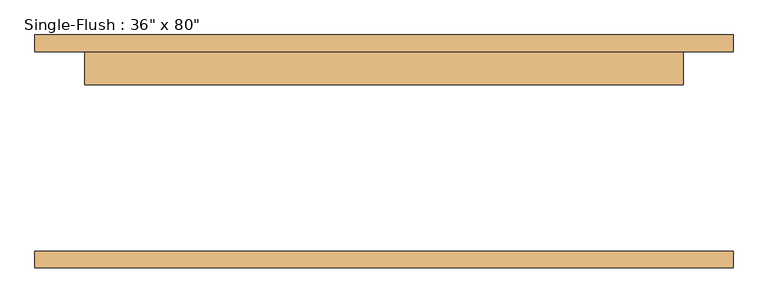
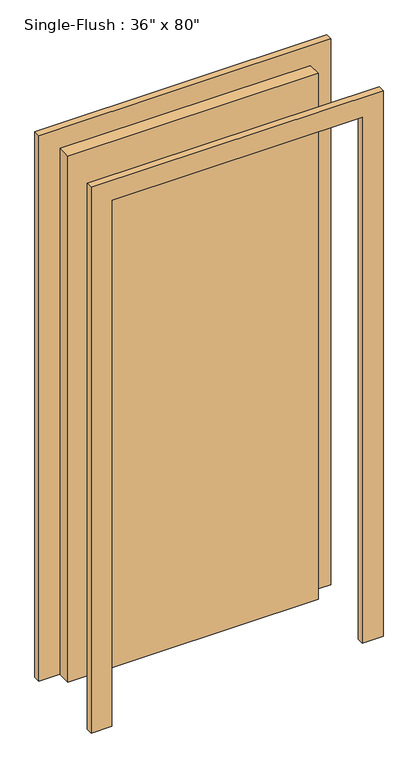
"""IFC4 building model written with IfcOpenShell, lengths in millimetres: door geometry."""

import ifcopenshell
import ifcopenshell.guid

model = None  # the IFC model being written
_history = None  # IfcOwnerHistory: only IFC2X3 demands one
_inside = {}  # id of a spatial element -> (the spatial element, [elements in it])
_under = {}  # id of a project, library or spatial element -> (it, [spatial elements below it])
_declared = {}  # id of a project -> (the project, [libraries it declares])
_typed = {}  # id of a type object -> (the type object, [elements of that type])
_made_of = {}  # id of a material, layer set ... -> (it, [elements and type objects made of it])


def new_model(schema):
    """Start an empty IFC model of exactly this schema.

    Asked for "IFC4X3", IfcOpenShell would pick the latest addendum, in which some entities
    have other attributes; the version numbers below select the first issue.
    IFC2X3 requires an IfcOwnerHistory on every rooted entity: one is made here for all.
    """
    global model, _history
    if schema == "IFC4X3":
        model = ifcopenshell.file(schema_version=(4, 3, 0, 0))
    else:
        model = ifcopenshell.file(schema=schema)
    _inside.clear()
    _under.clear()
    _declared.clear()
    _typed.clear()
    _made_of.clear()
    _history = None
    if model.schema == "IFC2X3":
        org = make("IfcOrganization", Name="unknown")
        user = make(
            "IfcPersonAndOrganization",
            ThePerson=make("IfcPerson", FamilyName="unknown"),
            TheOrganization=org,
        )
        app = make(
            "IfcApplication",
            ApplicationDeveloper=org,
            Version="unknown",
            ApplicationFullName="unknown",
            ApplicationIdentifier="unknown",
        )
        _history = make(
            "IfcOwnerHistory",
            OwningUser=user,
            OwningApplication=app,
            ChangeAction="ADDED",
            CreationDate=0,
        )
    return model


def make(cls, **values):
    """One entity of the class cls with the attributes given. An attribute that is None is left unset."""
    return model.create_entity(
        cls, **{name: value for name, value in values.items() if value is not None}
    )


def rooted(cls, **values):
    """An entity with a GlobalId (a new one), such as an element, a storey or a relation."""
    return make(cls, GlobalId=ifcopenshell.guid.new(), OwnerHistory=_history, **values)


def si_unit(unit_type, name, prefix=None):
    """IfcSIUnit, for example si_unit("LENGTHUNIT", "METRE", prefix="MILLI")."""
    return make("IfcSIUnit", UnitType=unit_type, Prefix=prefix, Name=name)


def assignment(units):
    """IfcUnitAssignment: the units of a project."""
    return None if units is None else make("IfcUnitAssignment", Units=units)


def point(xyz):
    """IfcCartesianPoint."""
    return None if xyz is None else make("IfcCartesianPoint", Coordinates=xyz)


def direction(xyz):
    """IfcDirection."""
    return None if xyz is None else make("IfcDirection", DirectionRatios=xyz)


def frame(location, z_axis=None, x_axis=None):
    """IfcAxis2Placement3D, a coordinate frame: its origin and axes. An axis left out is left unset."""
    return make(
        "IfcAxis2Placement3D",
        Location=point(location),
        Axis=direction(z_axis),
        RefDirection=direction(x_axis),
    )


def origin():
    """The frame at (0, 0, 0) with its axes left unset."""
    return frame((0.0, 0.0, 0.0))


def origin_with_axes():
    """The frame at (0, 0, 0) with the z axis (0, 0, 1) and the x axis (1, 0, 0) written out."""
    return frame((0.0, 0.0, 0.0), z_axis=(0.0, 0.0, 1.0), x_axis=(1.0, 0.0, 0.0))


def place(relative_to, where):
    """IfcLocalPlacement: puts the frame where relative to a parent placement (None: the world)."""
    return make(
        "IfcLocalPlacement", PlacementRelTo=relative_to, RelativePlacement=where
    )


def context(
    kind, dimensions, precision=None, world=None, true_north=None, identifier=None
):
    """IfcGeometricRepresentationContext, for example the 3D "Model" context."""
    return make(
        "IfcGeometricRepresentationContext",
        ContextIdentifier=identifier,
        ContextType=kind,
        CoordinateSpaceDimension=dimensions,
        Precision=precision,
        WorldCoordinateSystem=world,
        TrueNorth=true_north,
    )


def project(units=None, contexts=None):
    """IfcProject with its units and contexts."""
    return rooted(
        "IfcProject",
        Name="project",
        RepresentationContexts=contexts,
        UnitsInContext=assignment(units),
    )


def spatial(cls, under=None, at=None, **own):
    """A site, building, storey or space (cls), placed at a placement, below another one or the project."""
    s = rooted(cls, ObjectPlacement=at, **own)
    if under is not None:
        _under.setdefault(under.id(), (under, []))[1].append(s)
    return s


def polyline(points):
    """IfcPolyline through the points."""
    return make("IfcPolyline", Points=[point(p) for p in points])


def outline(outer, holes=None, kind="AREA"):
    """IfcArbitraryClosedProfileDef: a profile drawn as a closed curve; with holes, ...WithVoids."""
    if holes is None:
        return make("IfcArbitraryClosedProfileDef", ProfileType=kind, OuterCurve=outer)
    return make(
        "IfcArbitraryProfileDefWithVoids",
        ProfileType=kind,
        OuterCurve=outer,
        InnerCurves=holes,
    )


def extrude(swept, where, along, depth):
    """IfcExtrudedAreaSolid: the profile swept, set in the frame where, extruded along a direction by depth."""
    return make(
        "IfcExtrudedAreaSolid",
        SweptArea=swept,
        Position=where,
        ExtrudedDirection=direction(along),
        Depth=depth,
    )


def shape(context_of_items, identifier, shape_type, items):
    """IfcShapeRepresentation: the items that make up one representation, for example the "Body"."""
    return make(
        "IfcShapeRepresentation",
        ContextOfItems=context_of_items,
        RepresentationIdentifier=identifier,
        RepresentationType=shape_type,
        Items=items,
    )


def source(mapping_origin, context_of_items, identifier, shape_type, items):
    """IfcRepresentationMap: a shape defined once, which mapped items show again and again."""
    return make(
        "IfcRepresentationMap",
        MappingOrigin=mapping_origin,
        MappedRepresentation=shape(context_of_items, identifier, shape_type, items),
    )


def transform(
    local_origin,
    x_axis=None,
    y_axis=None,
    z_axis=None,
    scale=None,
    scale2=None,
    scale3=None,
    uniform=True,
):
    """IfcCartesianTransformationOperator3D, or its non-uniform kind. x_axis, y_axis, z_axis: its Axis1, 2, 3."""
    if uniform:
        return make(
            "IfcCartesianTransformationOperator3D",
            Axis1=direction(x_axis),
            Axis2=direction(y_axis),
            LocalOrigin=point(local_origin),
            Scale=scale,
            Axis3=direction(z_axis),
        )
    return make(
        "IfcCartesianTransformationOperator3DnonUniform",
        Axis1=direction(x_axis),
        Axis2=direction(y_axis),
        LocalOrigin=point(local_origin),
        Scale=scale,
        Axis3=direction(z_axis),
        Scale2=scale2,
        Scale3=scale3,
    )


def mapped(mapping_source, mapping_target):
    """IfcMappedItem: shows the shape of a source again, moved by a transform."""
    return make(
        "IfcMappedItem", MappingSource=mapping_source, MappingTarget=mapping_target
    )


def made_of(thing, what):
    """Note that an element or type object is made of a material, layer set ...; save() writes the relation."""
    if what is not None:
        _made_of.setdefault(what.id(), (what, []))[1].append(thing)
    return thing


def element(
    cls,
    number,
    at=None,
    inside=None,
    cuts=None,
    type_object=None,
    material=None,
    context=None,
    identifier="Body",
    shape_type=None,
    held_by="IfcProductDefinitionShape",
    body=None,
    shapes=None,
    **own,
):
    """One element of the class cls, such as IfcWall. Its Tag is "e" and its number.

    at: its placement. inside: the storey or other place that contains it. cuts: it is an
    opening in that element (IfcRelVoidsElement). A single representation is given by context,
    identifier, shape_type and body (its items); several are given by shapes. held_by: the class
    of the entity that holds the representations. save() writes the other relations.
    """
    e = rooted(cls, Tag="e%d" % number, ObjectPlacement=at, **own)
    if body is not None:
        shapes = [shape(context, identifier, shape_type, body)]
    if shapes is not None:
        e.Representation = make(held_by, Representations=shapes)
    if inside is not None:
        _inside.setdefault(inside.id(), (inside, []))[1].append(e)
    if cuts is not None:
        rooted(
            "IfcRelVoidsElement", RelatingBuildingElement=cuts, RelatedOpeningElement=e
        )
    if type_object is not None:
        _typed.setdefault(type_object.id(), (type_object, []))[1].append(e)
    return made_of(e, material)


def aggregate(whole, parts):
    """IfcRelAggregates: a whole, such as a stair, and the parts it consists of."""
    return rooted("IfcRelAggregates", RelatingObject=whole, RelatedObjects=parts)


def save(model, path):
    """Write the relations noted so far, then the file.

    IfcRelAggregates (storeys below a building ...), IfcRelContainedInSpatialStructure (elements
    in a storey), IfcRelDefinesByType, IfcRelAssociatesMaterial and IfcRelDeclares: one each for
    every whole, place, type object, material and project.
    """
    for whole, parts in _under.values():
        aggregate(whole, parts)
    for where, things in _inside.values():
        rooted(
            "IfcRelContainedInSpatialStructure",
            RelatedElements=things,
            RelatingStructure=where,
        )
    for kind, things in _typed.values():
        rooted("IfcRelDefinesByType", RelatedObjects=things, RelatingType=kind)
    for what, things in _made_of.values():
        rooted("IfcRelAssociatesMaterial", RelatedObjects=things, RelatingMaterial=what)
    for by, libraries in _declared.values():
        rooted("IfcRelDeclares", RelatingContext=by, RelatedDefinitions=libraries)
    model.write(path)


def door_efb18c7f(model_context):
    return source(origin(), model_context, "Body", "SweptSolid", [
        extrude(outline(polyline([(2108.2, -533.4), (0.0, -533.4), (0.0, -457.2), (2032.0, -457.2), (2032.0, 457.2), (0.0, 457.2), (0.0, 533.4), (2108.2, 533.4), (2108.2, -533.4)])), frame((0.0, 152.4, 0.0), z_axis=(0.0, 1.0, 0.0), x_axis=(0.0, 0.0, 1.0)), (0.0, 0.0, 1.0), 25.4),
        extrude(outline(polyline([(2108.2, 533.4), (2108.2, -533.4), (0.0, -533.4), (0.0, -457.2), (2032.0, -457.2), (2032.0, 457.2), (0.0, 457.2), (0.0, 533.4), (2108.2, 533.4)])), frame((0.0, -177.8, 0.0), z_axis=(0.0, 1.0, 0.0), x_axis=(0.0, 0.0, 1.0)), (0.0, 0.0, 1.0), 25.4),
        extrude(outline(polyline([(457.2, 101.6), (-457.2, 101.6), (-457.2, 152.4), (457.2, 152.4), (457.2, 101.6)])), origin_with_axes(), (0.0, 0.0, 1.0), 2032.0),
    ])


if __name__ == "__main__":
    model = new_model("IFC4")
    model_context = context("Model", 3, world=origin())
    ifc_project = project(units=[si_unit("LENGTHUNIT", "METRE", prefix="MILLI")], contexts=[model_context])
    site = spatial("IfcSite", under=ifc_project)
    building = spatial("IfcBuilding", under=site)
    placement = place(None, origin())
    door_shape = door_efb18c7f(model_context)
    element("IfcDoor", 1, ObjectType="Single-Flush : 36\" x 80\"", at=placement, inside=building, context=model_context, shape_type="MappedRepresentation", body=[
        mapped(door_shape, transform((0.0, 0.0, 0.0), x_axis=(1.0, 0.0, 0.0), y_axis=(0.0, 1.0, 0.0), z_axis=(0.0, 0.0, 1.0))),
    ])
    save(model, "model.ifc")

# Revit data of these elements
# Type "Single-Flush : 36\" x 80\""
#   Type Mark = "6"
#   Construction Type Id = "MDOOR"
#   Assembly Code = "C1020"
#   Analytic Construction = "Metal"
#   Thickness = 0' - 2"
#   Heat Transfer Coefficient (U) = 0.651978 BTU/(h·ft²·°F)
#   Height = 6' - 8"
#   Trim Projection Ext = 0' - 1"
#   Trim Projection Int = 0' - 1"
#   Trim Width = 0' - 3"
#   Width = 3' - 0"
#   Define Thermal Properties by = 1
#   Define Thermal Properties by = 1
#   Door Material = Door - Panel
#   Frame Material = Door - Frame
#   Visual Light Transmittance = 0
#   Solar Heat Gain Coefficient = 0
#   Function = (empty or 0)
#   Wall Closure = (empty or 0)
# Element 1 (IfcDoor, "Single-Flush : 36\" x 80\"")
#   Materials on its faces: "Door - Frame", "Door - Panel"
# Materials
#   "Door - Panel": class "Wood", colour RGB 210 159 95, transparency 0, Cost = 0
#   "Door - Frame": class "Miscellaneous", colour RGB 118 70 51, transparency 0, Cost = 0
